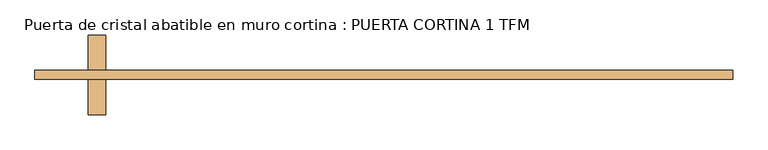
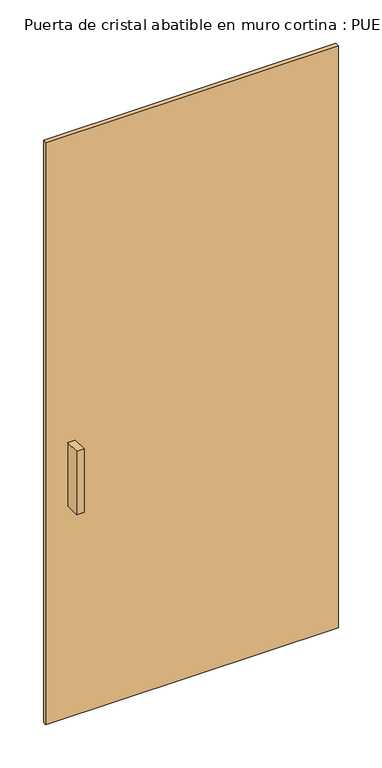
"""IFC4 building model written with IfcOpenShell, lengths in millimetres: door geometry, Puerta de cristal abatible en muro cortina : PUERTA CORTINA 1 TFM."""

import ifcopenshell
import ifcopenshell.guid

model = None  # the IFC model being written
_history = None  # IfcOwnerHistory: only IFC2X3 demands one
_inside = {}  # id of a spatial element -> (the spatial element, [elements in it])
_under = {}  # id of a project, library or spatial element -> (it, [spatial elements below it])
_declared = {}  # id of a project -> (the project, [libraries it declares])
_typed = {}  # id of a type object -> (the type object, [elements of that type])
_made_of = {}  # id of a material, layer set ... -> (it, [elements and type objects made of it])


def new_model(schema):
    """Start an empty IFC model of exactly this schema.

    Asked for "IFC4X3", IfcOpenShell would pick the latest addendum, in which some entities
    have other attributes; the version numbers below select the first issue.
    IFC2X3 requires an IfcOwnerHistory on every rooted entity: one is made here for all.
    """
    global model, _history
    if schema == "IFC4X3":
        model = ifcopenshell.file(schema_version=(4, 3, 0, 0))
    else:
        model = ifcopenshell.file(schema=schema)
    _inside.clear()
    _under.clear()
    _declared.clear()
    _typed.clear()
    _made_of.clear()
    _history = None
    if model.schema == "IFC2X3":
        org = make("IfcOrganization", Name="unknown")
        user = make(
            "IfcPersonAndOrganization",
            ThePerson=make("IfcPerson", FamilyName="unknown"),
            TheOrganization=org,
        )
        app = make(
            "IfcApplication",
            ApplicationDeveloper=org,
            Version="unknown",
            ApplicationFullName="unknown",
            ApplicationIdentifier="unknown",
        )
        _history = make(
            "IfcOwnerHistory",
            OwningUser=user,
            OwningApplication=app,
            ChangeAction="ADDED",
            CreationDate=0,
        )
    return model


def make(cls, **values):
    """One entity of the class cls with the attributes given. An attribute that is None is left unset."""
    return model.create_entity(
        cls, **{name: value for name, value in values.items() if value is not None}
    )


def rooted(cls, **values):
    """An entity with a GlobalId (a new one), such as an element, a storey or a relation."""
    return make(cls, GlobalId=ifcopenshell.guid.new(), OwnerHistory=_history, **values)


def si_unit(unit_type, name, prefix=None):
    """IfcSIUnit, for example si_unit("LENGTHUNIT", "METRE", prefix="MILLI")."""
    return make("IfcSIUnit", UnitType=unit_type, Prefix=prefix, Name=name)


def assignment(units):
    """IfcUnitAssignment: the units of a project."""
    return None if units is None else make("IfcUnitAssignment", Units=units)


def point(xyz):
    """IfcCartesianPoint."""
    return None if xyz is None else make("IfcCartesianPoint", Coordinates=xyz)


def direction(xyz):
    """IfcDirection."""
    return None if xyz is None else make("IfcDirection", DirectionRatios=xyz)


def frame(location, z_axis=None, x_axis=None):
    """IfcAxis2Placement3D, a coordinate frame: its origin and axes. An axis left out is left unset."""
    return make(
        "IfcAxis2Placement3D",
        Location=point(location),
        Axis=direction(z_axis),
        RefDirection=direction(x_axis),
    )


def origin():
    """The frame at (0, 0, 0) with its axes left unset."""
    return frame((0.0, 0.0, 0.0))


def origin_with_axes():
    """The frame at (0, 0, 0) with the z axis (0, 0, 1) and the x axis (1, 0, 0) written out."""
    return frame((0.0, 0.0, 0.0), z_axis=(0.0, 0.0, 1.0), x_axis=(1.0, 0.0, 0.0))


def place(relative_to, where):
    """IfcLocalPlacement: puts the frame where relative to a parent placement (None: the world)."""
    return make(
        "IfcLocalPlacement", PlacementRelTo=relative_to, RelativePlacement=where
    )


def context(
    kind, dimensions, precision=None, world=None, true_north=None, identifier=None
):
    """IfcGeometricRepresentationContext, for example the 3D "Model" context."""
    return make(
        "IfcGeometricRepresentationContext",
        ContextIdentifier=identifier,
        ContextType=kind,
        CoordinateSpaceDimension=dimensions,
        Precision=precision,
        WorldCoordinateSystem=world,
        TrueNorth=true_north,
    )


def project(units=None, contexts=None):
    """IfcProject with its units and contexts."""
    return rooted(
        "IfcProject",
        Name="project",
        RepresentationContexts=contexts,
        UnitsInContext=assignment(units),
    )


def spatial(cls, under=None, at=None, **own):
    """A site, building, storey or space (cls), placed at a placement, below another one or the project."""
    s = rooted(cls, ObjectPlacement=at, **own)
    if under is not None:
        _under.setdefault(under.id(), (under, []))[1].append(s)
    return s


def polyline(points):
    """IfcPolyline through the points."""
    return make("IfcPolyline", Points=[point(p) for p in points])


def outline(outer, holes=None, kind="AREA"):
    """IfcArbitraryClosedProfileDef: a profile drawn as a closed curve; with holes, ...WithVoids."""
    if holes is None:
        return make("IfcArbitraryClosedProfileDef", ProfileType=kind, OuterCurve=outer)
    return make(
        "IfcArbitraryProfileDefWithVoids",
        ProfileType=kind,
        OuterCurve=outer,
        InnerCurves=holes,
    )


def extrude(swept, where, along, depth):
    """IfcExtrudedAreaSolid: the profile swept, set in the frame where, extruded along a direction by depth."""
    return make(
        "IfcExtrudedAreaSolid",
        SweptArea=swept,
        Position=where,
        ExtrudedDirection=direction(along),
        Depth=depth,
    )


def shape(context_of_items, identifier, shape_type, items):
    """IfcShapeRepresentation: the items that make up one representation, for example the "Body"."""
    return make(
        "IfcShapeRepresentation",
        ContextOfItems=context_of_items,
        RepresentationIdentifier=identifier,
        RepresentationType=shape_type,
        Items=items,
    )


def source(mapping_origin, context_of_items, identifier, shape_type, items):
    """IfcRepresentationMap: a shape defined once, which mapped items show again and again."""
    return make(
        "IfcRepresentationMap",
        MappingOrigin=mapping_origin,
        MappedRepresentation=shape(context_of_items, identifier, shape_type, items),
    )


def transform(
    local_origin,
    x_axis=None,
    y_axis=None,
    z_axis=None,
    scale=None,
    scale2=None,
    scale3=None,
    uniform=True,
):
    """IfcCartesianTransformationOperator3D, or its non-uniform kind. x_axis, y_axis, z_axis: its Axis1, 2, 3."""
    if uniform:
        return make(
            "IfcCartesianTransformationOperator3D",
            Axis1=direction(x_axis),
            Axis2=direction(y_axis),
            LocalOrigin=point(local_origin),
            Scale=scale,
            Axis3=direction(z_axis),
        )
    return make(
        "IfcCartesianTransformationOperator3DnonUniform",
        Axis1=direction(x_axis),
        Axis2=direction(y_axis),
        LocalOrigin=point(local_origin),
        Scale=scale,
        Axis3=direction(z_axis),
        Scale2=scale2,
        Scale3=scale3,
    )


def mapped(mapping_source, mapping_target):
    """IfcMappedItem: shows the shape of a source again, moved by a transform."""
    return make(
        "IfcMappedItem", MappingSource=mapping_source, MappingTarget=mapping_target
    )


def made_of(thing, what):
    """Note that an element or type object is made of a material, layer set ...; save() writes the relation."""
    if what is not None:
        _made_of.setdefault(what.id(), (what, []))[1].append(thing)
    return thing


def element(
    cls,
    number,
    at=None,
    inside=None,
    cuts=None,
    type_object=None,
    material=None,
    context=None,
    identifier="Body",
    shape_type=None,
    held_by="IfcProductDefinitionShape",
    body=None,
    shapes=None,
    **own,
):
    """One element of the class cls, such as IfcWall. Its Tag is "e" and its number.

    at: its placement. inside: the storey or other place that contains it. cuts: it is an
    opening in that element (IfcRelVoidsElement). A single representation is given by context,
    identifier, shape_type and body (its items); several are given by shapes. held_by: the class
    of the entity that holds the representations. save() writes the other relations.
    """
    e = rooted(cls, Tag="e%d" % number, ObjectPlacement=at, **own)
    if body is not None:
        shapes = [shape(context, identifier, shape_type, body)]
    if shapes is not None:
        e.Representation = make(held_by, Representations=shapes)
    if inside is not None:
        _inside.setdefault(inside.id(), (inside, []))[1].append(e)
    if cuts is not None:
        rooted(
            "IfcRelVoidsElement", RelatingBuildingElement=cuts, RelatedOpeningElement=e
        )
    if type_object is not None:
        _typed.setdefault(type_object.id(), (type_object, []))[1].append(e)
    return made_of(e, material)


def aggregate(whole, parts):
    """IfcRelAggregates: a whole, such as a stair, and the parts it consists of."""
    return rooted("IfcRelAggregates", RelatingObject=whole, RelatedObjects=parts)


def save(model, path):
    """Write the relations noted so far, then the file.

    IfcRelAggregates (storeys below a building ...), IfcRelContainedInSpatialStructure (elements
    in a storey), IfcRelDefinesByType, IfcRelAssociatesMaterial and IfcRelDeclares: one each for
    every whole, place, type object, material and project.
    """
    for whole, parts in _under.values():
        aggregate(whole, parts)
    for where, things in _inside.values():
        rooted(
            "IfcRelContainedInSpatialStructure",
            RelatedElements=things,
            RelatingStructure=where,
        )
    for kind, things in _typed.values():
        rooted("IfcRelDefinesByType", RelatedObjects=things, RelatingType=kind)
    for what, things in _made_of.values():
        rooted("IfcRelAssociatesMaterial", RelatedObjects=things, RelatingMaterial=what)
    for by, libraries in _declared.values():
        rooted("IfcRelDeclares", RelatingContext=by, RelatedDefinitions=libraries)
    model.write(path)


def puerta_de_cristal_abatible_en_muro_cortina_puerta_cortina_1_2cb0721c(model_context):
    return source(origin(), model_context, "Body", "SweptSolid", [
        extrude(outline(polyline([(-398.4, -12.5), (-423.8, -12.5), (-423.8, 38.3), (-398.4, 38.3), (-398.4, -12.5)])), frame((0.0, 0.0, 762.0), z_axis=(0.0, 0.0, 1.0), x_axis=(1.0, 0.0, 0.0)), (0.0, 0.0, 1.0), 228.6),
        extrude(outline(polyline([(-423.8, 101.8), (-398.4, 101.8), (-398.4, 51.0), (-423.8, 51.0), (-423.8, 101.8)])), frame((0.0, 0.0, 762.0), z_axis=(0.0, 0.0, 1.0), x_axis=(1.0, 0.0, 0.0)), (0.0, 0.0, 1.0), 228.6),
        extrude(outline(polyline([(500.0, 51.0), (500.0, 38.3), (-500.0, 38.3), (-500.0, 51.0), (500.0, 51.0)])), origin_with_axes(), (0.0, 0.0, 1.0), 2100.0),
    ])


if __name__ == "__main__":
    model = new_model("IFC4")
    model_context = context("Model", 3, world=origin())
    ifc_project = project(units=[si_unit("LENGTHUNIT", "METRE", prefix="MILLI")], contexts=[model_context])
    site = spatial("IfcSite", under=ifc_project)
    building = spatial("IfcBuilding", under=site)
    placement = place(None, origin())
    puerta_de_cristal_abatible_en_muro_cortina_puerta_cortina_1_shape = puerta_de_cristal_abatible_en_muro_cortina_puerta_cortina_1_2cb0721c(model_context)
    element("IfcDoor", 1, ObjectType="Puerta de cristal abatible en muro cortina : PUERTA CORTINA 1 TFM", at=placement, inside=building, context=model_context, shape_type="MappedRepresentation", body=[
        mapped(puerta_de_cristal_abatible_en_muro_cortina_puerta_cortina_1_shape, transform((0.0, 0.0, 0.0), x_axis=(1.0, 0.0, 0.0), y_axis=(0.0, 1.0, 0.0), z_axis=(0.0, 0.0, 1.0))),
    ])
    save(model, "model.ifc")

# Revit data of these elements
# Type "Puerta de cristal abatible en muro cortina : PUERTA CORTINA 1 TFM"
#   Description = "Puerta vidrio muro cortina"
#   Type Mark = "P4"
#   Construction Type Id = "SGL"
#   Analytic Construction = "Ventanas grandes con acristalamiento simple"
#   Visual Light Transmittance = 0.9
#   Solar Heat Gain Coefficient = 0.86
#   Desfase = 0.051 m
#   Heat Transfer Coefficient (U) = 5.5617 W/(m²·K)
#   Define Thermal Properties by = 1
#   Function = 1
#   Material de cristalera = Vidrio
# Element 1 (IfcDoor, "Puerta de cristal abatible en muro cortina : PUERTA CORTINA 1 TFM")
#   Materials on its faces: "Metal - Aluminio", "Vidrio"
# Materials
#   "Vidrio": class "Vidrio", colour RGB 0 128 192, transparency 0.75, Description = "Vidrio de cal sodada", Cost = 0
#   "Metal - Aluminio": class "Metal", colour RGB 247 247 247, transparency 0
